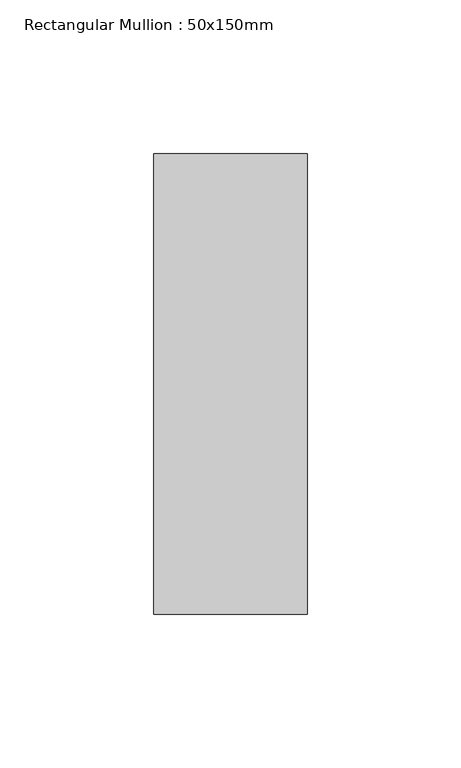
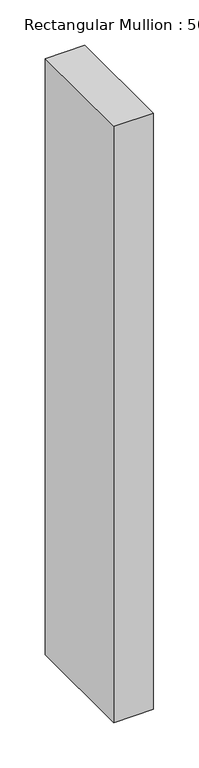
"""IFC4 building model written with IfcOpenShell, lengths in millimetres: member geometry, Rectangular Mullion : 50x150mm."""

import ifcopenshell
import ifcopenshell.guid

model = None  # the IFC model being written
_history = None  # IfcOwnerHistory: only IFC2X3 demands one
_inside = {}  # id of a spatial element -> (the spatial element, [elements in it])
_under = {}  # id of a project, library or spatial element -> (it, [spatial elements below it])
_declared = {}  # id of a project -> (the project, [libraries it declares])
_typed = {}  # id of a type object -> (the type object, [elements of that type])
_made_of = {}  # id of a material, layer set ... -> (it, [elements and type objects made of it])


def new_model(schema):
    """Start an empty IFC model of exactly this schema.

    Asked for "IFC4X3", IfcOpenShell would pick the latest addendum, in which some entities
    have other attributes; the version numbers below select the first issue.
    IFC2X3 requires an IfcOwnerHistory on every rooted entity: one is made here for all.
    """
    global model, _history
    if schema == "IFC4X3":
        model = ifcopenshell.file(schema_version=(4, 3, 0, 0))
    else:
        model = ifcopenshell.file(schema=schema)
    _inside.clear()
    _under.clear()
    _declared.clear()
    _typed.clear()
    _made_of.clear()
    _history = None
    if model.schema == "IFC2X3":
        org = make("IfcOrganization", Name="unknown")
        user = make(
            "IfcPersonAndOrganization",
            ThePerson=make("IfcPerson", FamilyName="unknown"),
            TheOrganization=org,
        )
        app = make(
            "IfcApplication",
            ApplicationDeveloper=org,
            Version="unknown",
            ApplicationFullName="unknown",
            ApplicationIdentifier="unknown",
        )
        _history = make(
            "IfcOwnerHistory",
            OwningUser=user,
            OwningApplication=app,
            ChangeAction="ADDED",
            CreationDate=0,
        )
    return model


def make(cls, **values):
    """One entity of the class cls with the attributes given. An attribute that is None is left unset."""
    return model.create_entity(
        cls, **{name: value for name, value in values.items() if value is not None}
    )


def rooted(cls, **values):
    """An entity with a GlobalId (a new one), such as an element, a storey or a relation."""
    return make(cls, GlobalId=ifcopenshell.guid.new(), OwnerHistory=_history, **values)


def si_unit(unit_type, name, prefix=None):
    """IfcSIUnit, for example si_unit("LENGTHUNIT", "METRE", prefix="MILLI")."""
    return make("IfcSIUnit", UnitType=unit_type, Prefix=prefix, Name=name)


def assignment(units):
    """IfcUnitAssignment: the units of a project."""
    return None if units is None else make("IfcUnitAssignment", Units=units)


def point(xyz):
    """IfcCartesianPoint."""
    return None if xyz is None else make("IfcCartesianPoint", Coordinates=xyz)


def direction(xyz):
    """IfcDirection."""
    return None if xyz is None else make("IfcDirection", DirectionRatios=xyz)


def frame(location, z_axis=None, x_axis=None):
    """IfcAxis2Placement3D, a coordinate frame: its origin and axes. An axis left out is left unset."""
    return make(
        "IfcAxis2Placement3D",
        Location=point(location),
        Axis=direction(z_axis),
        RefDirection=direction(x_axis),
    )


def origin():
    """The frame at (0, 0, 0) with its axes left unset."""
    return frame((0.0, 0.0, 0.0))


def place(relative_to, where):
    """IfcLocalPlacement: puts the frame where relative to a parent placement (None: the world)."""
    return make(
        "IfcLocalPlacement", PlacementRelTo=relative_to, RelativePlacement=where
    )


def context(
    kind, dimensions, precision=None, world=None, true_north=None, identifier=None
):
    """IfcGeometricRepresentationContext, for example the 3D "Model" context."""
    return make(
        "IfcGeometricRepresentationContext",
        ContextIdentifier=identifier,
        ContextType=kind,
        CoordinateSpaceDimension=dimensions,
        Precision=precision,
        WorldCoordinateSystem=world,
        TrueNorth=true_north,
    )


def project(units=None, contexts=None):
    """IfcProject with its units and contexts."""
    return rooted(
        "IfcProject",
        Name="project",
        RepresentationContexts=contexts,
        UnitsInContext=assignment(units),
    )


def spatial(cls, under=None, at=None, **own):
    """A site, building, storey or space (cls), placed at a placement, below another one or the project."""
    s = rooted(cls, ObjectPlacement=at, **own)
    if under is not None:
        _under.setdefault(under.id(), (under, []))[1].append(s)
    return s


def polyline(points):
    """IfcPolyline through the points."""
    return make("IfcPolyline", Points=[point(p) for p in points])


def outline(outer, holes=None, kind="AREA"):
    """IfcArbitraryClosedProfileDef: a profile drawn as a closed curve; with holes, ...WithVoids."""
    if holes is None:
        return make("IfcArbitraryClosedProfileDef", ProfileType=kind, OuterCurve=outer)
    return make(
        "IfcArbitraryProfileDefWithVoids",
        ProfileType=kind,
        OuterCurve=outer,
        InnerCurves=holes,
    )


def extrude(swept, where, along, depth):
    """IfcExtrudedAreaSolid: the profile swept, set in the frame where, extruded along a direction by depth."""
    return make(
        "IfcExtrudedAreaSolid",
        SweptArea=swept,
        Position=where,
        ExtrudedDirection=direction(along),
        Depth=depth,
    )


def shape(context_of_items, identifier, shape_type, items):
    """IfcShapeRepresentation: the items that make up one representation, for example the "Body"."""
    return make(
        "IfcShapeRepresentation",
        ContextOfItems=context_of_items,
        RepresentationIdentifier=identifier,
        RepresentationType=shape_type,
        Items=items,
    )


def source(mapping_origin, context_of_items, identifier, shape_type, items):
    """IfcRepresentationMap: a shape defined once, which mapped items show again and again."""
    return make(
        "IfcRepresentationMap",
        MappingOrigin=mapping_origin,
        MappedRepresentation=shape(context_of_items, identifier, shape_type, items),
    )


def transform(
    local_origin,
    x_axis=None,
    y_axis=None,
    z_axis=None,
    scale=None,
    scale2=None,
    scale3=None,
    uniform=True,
):
    """IfcCartesianTransformationOperator3D, or its non-uniform kind. x_axis, y_axis, z_axis: its Axis1, 2, 3."""
    if uniform:
        return make(
            "IfcCartesianTransformationOperator3D",
            Axis1=direction(x_axis),
            Axis2=direction(y_axis),
            LocalOrigin=point(local_origin),
            Scale=scale,
            Axis3=direction(z_axis),
        )
    return make(
        "IfcCartesianTransformationOperator3DnonUniform",
        Axis1=direction(x_axis),
        Axis2=direction(y_axis),
        LocalOrigin=point(local_origin),
        Scale=scale,
        Axis3=direction(z_axis),
        Scale2=scale2,
        Scale3=scale3,
    )


def mapped(mapping_source, mapping_target):
    """IfcMappedItem: shows the shape of a source again, moved by a transform."""
    return make(
        "IfcMappedItem", MappingSource=mapping_source, MappingTarget=mapping_target
    )


def made_of(thing, what):
    """Note that an element or type object is made of a material, layer set ...; save() writes the relation."""
    if what is not None:
        _made_of.setdefault(what.id(), (what, []))[1].append(thing)
    return thing


def element(
    cls,
    number,
    at=None,
    inside=None,
    cuts=None,
    type_object=None,
    material=None,
    context=None,
    identifier="Body",
    shape_type=None,
    held_by="IfcProductDefinitionShape",
    body=None,
    shapes=None,
    **own,
):
    """One element of the class cls, such as IfcWall. Its Tag is "e" and its number.

    at: its placement. inside: the storey or other place that contains it. cuts: it is an
    opening in that element (IfcRelVoidsElement). A single representation is given by context,
    identifier, shape_type and body (its items); several are given by shapes. held_by: the class
    of the entity that holds the representations. save() writes the other relations.
    """
    e = rooted(cls, Tag="e%d" % number, ObjectPlacement=at, **own)
    if body is not None:
        shapes = [shape(context, identifier, shape_type, body)]
    if shapes is not None:
        e.Representation = make(held_by, Representations=shapes)
    if inside is not None:
        _inside.setdefault(inside.id(), (inside, []))[1].append(e)
    if cuts is not None:
        rooted(
            "IfcRelVoidsElement", RelatingBuildingElement=cuts, RelatedOpeningElement=e
        )
    if type_object is not None:
        _typed.setdefault(type_object.id(), (type_object, []))[1].append(e)
    return made_of(e, material)


def aggregate(whole, parts):
    """IfcRelAggregates: a whole, such as a stair, and the parts it consists of."""
    return rooted("IfcRelAggregates", RelatingObject=whole, RelatedObjects=parts)


def save(model, path):
    """Write the relations noted so far, then the file.

    IfcRelAggregates (storeys below a building ...), IfcRelContainedInSpatialStructure (elements
    in a storey), IfcRelDefinesByType, IfcRelAssociatesMaterial and IfcRelDeclares: one each for
    every whole, place, type object, material and project.
    """
    for whole, parts in _under.values():
        aggregate(whole, parts)
    for where, things in _inside.values():
        rooted(
            "IfcRelContainedInSpatialStructure",
            RelatedElements=things,
            RelatingStructure=where,
        )
    for kind, things in _typed.values():
        rooted("IfcRelDefinesByType", RelatedObjects=things, RelatingType=kind)
    for what, things in _made_of.values():
        rooted("IfcRelAssociatesMaterial", RelatedObjects=things, RelatingMaterial=what)
    for by, libraries in _declared.values():
        rooted("IfcRelDeclares", RelatingContext=by, RelatedDefinitions=libraries)
    model.write(path)


def rectangular_mullion_50x150mm_6ffebc0f(model_context):
    return source(origin(), model_context, "Body", "SweptSolid", [
        extrude(outline(polyline([(0.0, 75.0), (0.0, -75.0), (-50.0, -75.0), (-50.0, 75.0), (0.0, 75.0)])), frame((0.0, 0.0, -800.0), z_axis=(0.0, 0.0, 1.0), x_axis=(1.0, 0.0, 0.0)), (0.0, 0.0, 1.0), 800.0),
    ])


if __name__ == "__main__":
    model = new_model("IFC4")
    model_context = context("Model", 3, world=origin())
    ifc_project = project(units=[si_unit("LENGTHUNIT", "METRE", prefix="MILLI")], contexts=[model_context])
    site = spatial("IfcSite", under=ifc_project)
    building = spatial("IfcBuilding", under=site)
    placement = place(None, origin())
    rectangular_mullion_50x150mm_shape = rectangular_mullion_50x150mm_6ffebc0f(model_context)
    element("IfcMember", 1, ObjectType="Rectangular Mullion : 50x150mm", at=placement, inside=building, context=model_context, shape_type="MappedRepresentation", body=[
        mapped(rectangular_mullion_50x150mm_shape, transform((0.0, 0.0, 0.0), x_axis=(1.0, 0.0, 0.0), y_axis=(0.0, 1.0, 0.0), z_axis=(0.0, 0.0, 1.0))),
    ])
    save(model, "model.ifc")

# Revit data of these elements
# Project information
#   Project Issue Date = "Issue Date"
#   Project Status = "Project Status"
#   Client Name = "Owner"
#   Project Address = "Enter address here"
#   Project Name = "Project Name"
#   Project Number = "Project Number"
# Type "Rectangular Mullion : 50x150mm"
#   Keynote = "H11"
#   built-in parameter 1007304 = 0.492126 (stored number, unit not read)
#   built-in parameter 1007301 = 0.082021 (stored number, unit not read)
#   built-in parameter 1007300 = 0.082021 (stored number, unit not read)
# Element 1 (IfcMember, "Rectangular Mullion : 50x150mm")
#   Materials on its faces: "Aluminium"
# Materials
#   "Aluminium": class "Metal", colour RGB 247 247 247, transparency 0, Description = "Aluminium 6061", Cost = 0
